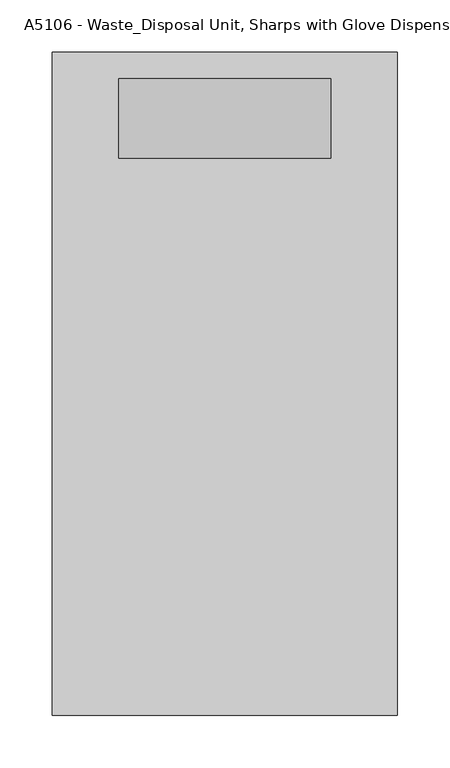
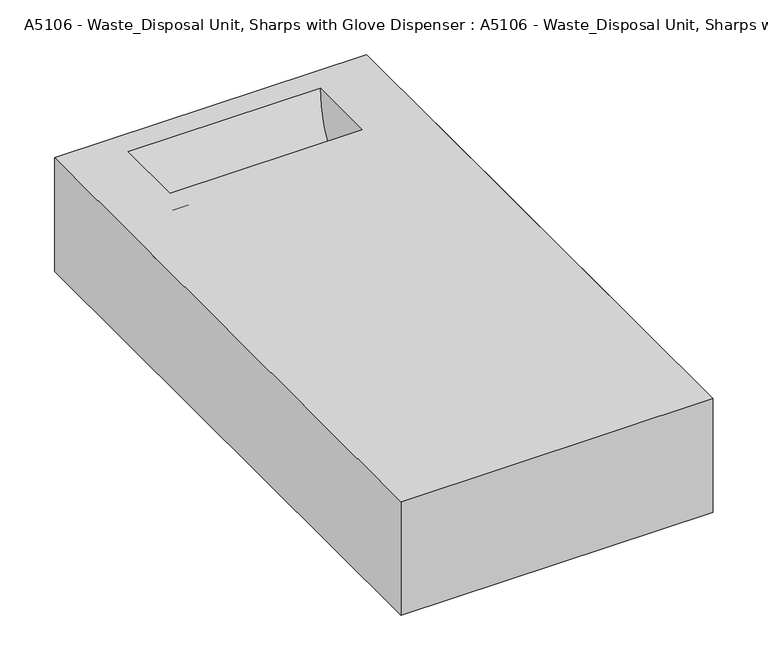
"""IFC4 building model written with IfcOpenShell, lengths in millimetres: proxy geometry, A5106 - Waste_Disposal Unit, Sharps with Glove Dispenser : A5106 - Waste_Disposal Unit, Sharps with Glove Dispenser."""

import ifcopenshell
import ifcopenshell.guid

model = None  # the IFC model being written
_history = None  # IfcOwnerHistory: only IFC2X3 demands one
_inside = {}  # id of a spatial element -> (the spatial element, [elements in it])
_under = {}  # id of a project, library or spatial element -> (it, [spatial elements below it])
_declared = {}  # id of a project -> (the project, [libraries it declares])
_typed = {}  # id of a type object -> (the type object, [elements of that type])
_made_of = {}  # id of a material, layer set ... -> (it, [elements and type objects made of it])


def new_model(schema):
    """Start an empty IFC model of exactly this schema.

    Asked for "IFC4X3", IfcOpenShell would pick the latest addendum, in which some entities
    have other attributes; the version numbers below select the first issue.
    IFC2X3 requires an IfcOwnerHistory on every rooted entity: one is made here for all.
    """
    global model, _history
    if schema == "IFC4X3":
        model = ifcopenshell.file(schema_version=(4, 3, 0, 0))
    else:
        model = ifcopenshell.file(schema=schema)
    _inside.clear()
    _under.clear()
    _declared.clear()
    _typed.clear()
    _made_of.clear()
    _history = None
    if model.schema == "IFC2X3":
        org = make("IfcOrganization", Name="unknown")
        user = make(
            "IfcPersonAndOrganization",
            ThePerson=make("IfcPerson", FamilyName="unknown"),
            TheOrganization=org,
        )
        app = make(
            "IfcApplication",
            ApplicationDeveloper=org,
            Version="unknown",
            ApplicationFullName="unknown",
            ApplicationIdentifier="unknown",
        )
        _history = make(
            "IfcOwnerHistory",
            OwningUser=user,
            OwningApplication=app,
            ChangeAction="ADDED",
            CreationDate=0,
        )
    return model


def make(cls, **values):
    """One entity of the class cls with the attributes given. An attribute that is None is left unset."""
    return model.create_entity(
        cls, **{name: value for name, value in values.items() if value is not None}
    )


def rooted(cls, **values):
    """An entity with a GlobalId (a new one), such as an element, a storey or a relation."""
    return make(cls, GlobalId=ifcopenshell.guid.new(), OwnerHistory=_history, **values)


def si_unit(unit_type, name, prefix=None):
    """IfcSIUnit, for example si_unit("LENGTHUNIT", "METRE", prefix="MILLI")."""
    return make("IfcSIUnit", UnitType=unit_type, Prefix=prefix, Name=name)


def assignment(units):
    """IfcUnitAssignment: the units of a project."""
    return None if units is None else make("IfcUnitAssignment", Units=units)


def point(xyz):
    """IfcCartesianPoint."""
    return None if xyz is None else make("IfcCartesianPoint", Coordinates=xyz)


def direction(xyz):
    """IfcDirection."""
    return None if xyz is None else make("IfcDirection", DirectionRatios=xyz)


def frame(location, z_axis=None, x_axis=None):
    """IfcAxis2Placement3D, a coordinate frame: its origin and axes. An axis left out is left unset."""
    return make(
        "IfcAxis2Placement3D",
        Location=point(location),
        Axis=direction(z_axis),
        RefDirection=direction(x_axis),
    )


def origin():
    """The frame at (0, 0, 0) with its axes left unset."""
    return frame((0.0, 0.0, 0.0))


def origin_with_axes():
    """The frame at (0, 0, 0) with the z axis (0, 0, 1) and the x axis (1, 0, 0) written out."""
    return frame((0.0, 0.0, 0.0), z_axis=(0.0, 0.0, 1.0), x_axis=(1.0, 0.0, 0.0))


def place(relative_to, where):
    """IfcLocalPlacement: puts the frame where relative to a parent placement (None: the world)."""
    return make(
        "IfcLocalPlacement", PlacementRelTo=relative_to, RelativePlacement=where
    )


def context(
    kind, dimensions, precision=None, world=None, true_north=None, identifier=None
):
    """IfcGeometricRepresentationContext, for example the 3D "Model" context."""
    return make(
        "IfcGeometricRepresentationContext",
        ContextIdentifier=identifier,
        ContextType=kind,
        CoordinateSpaceDimension=dimensions,
        Precision=precision,
        WorldCoordinateSystem=world,
        TrueNorth=true_north,
    )


def project(units=None, contexts=None):
    """IfcProject with its units and contexts."""
    return rooted(
        "IfcProject",
        Name="project",
        RepresentationContexts=contexts,
        UnitsInContext=assignment(units),
    )


def spatial(cls, under=None, at=None, **own):
    """A site, building, storey or space (cls), placed at a placement, below another one or the project."""
    s = rooted(cls, ObjectPlacement=at, **own)
    if under is not None:
        _under.setdefault(under.id(), (under, []))[1].append(s)
    return s


def polyline(points):
    """IfcPolyline through the points."""
    return make("IfcPolyline", Points=[point(p) for p in points])


def circle_curve(where, radius):
    """IfcCircle in the frame where."""
    return make("IfcCircle", Position=where, Radius=radius)


def outline(outer, holes=None, kind="AREA"):
    """IfcArbitraryClosedProfileDef: a profile drawn as a closed curve; with holes, ...WithVoids."""
    if holes is None:
        return make("IfcArbitraryClosedProfileDef", ProfileType=kind, OuterCurve=outer)
    return make(
        "IfcArbitraryProfileDefWithVoids",
        ProfileType=kind,
        OuterCurve=outer,
        InnerCurves=holes,
    )


def extrude(swept, where, along, depth):
    """IfcExtrudedAreaSolid: the profile swept, set in the frame where, extruded along a direction by depth."""
    return make(
        "IfcExtrudedAreaSolid",
        SweptArea=swept,
        Position=where,
        ExtrudedDirection=direction(along),
        Depth=depth,
    )


def shape(context_of_items, identifier, shape_type, items):
    """IfcShapeRepresentation: the items that make up one representation, for example the "Body"."""
    return make(
        "IfcShapeRepresentation",
        ContextOfItems=context_of_items,
        RepresentationIdentifier=identifier,
        RepresentationType=shape_type,
        Items=items,
    )


def source(mapping_origin, context_of_items, identifier, shape_type, items):
    """IfcRepresentationMap: a shape defined once, which mapped items show again and again."""
    return make(
        "IfcRepresentationMap",
        MappingOrigin=mapping_origin,
        MappedRepresentation=shape(context_of_items, identifier, shape_type, items),
    )


def transform(
    local_origin,
    x_axis=None,
    y_axis=None,
    z_axis=None,
    scale=None,
    scale2=None,
    scale3=None,
    uniform=True,
):
    """IfcCartesianTransformationOperator3D, or its non-uniform kind. x_axis, y_axis, z_axis: its Axis1, 2, 3."""
    if uniform:
        return make(
            "IfcCartesianTransformationOperator3D",
            Axis1=direction(x_axis),
            Axis2=direction(y_axis),
            LocalOrigin=point(local_origin),
            Scale=scale,
            Axis3=direction(z_axis),
        )
    return make(
        "IfcCartesianTransformationOperator3DnonUniform",
        Axis1=direction(x_axis),
        Axis2=direction(y_axis),
        LocalOrigin=point(local_origin),
        Scale=scale,
        Axis3=direction(z_axis),
        Scale2=scale2,
        Scale3=scale3,
    )


def mapped(mapping_source, mapping_target):
    """IfcMappedItem: shows the shape of a source again, moved by a transform."""
    return make(
        "IfcMappedItem", MappingSource=mapping_source, MappingTarget=mapping_target
    )


def made_of(thing, what):
    """Note that an element or type object is made of a material, layer set ...; save() writes the relation."""
    if what is not None:
        _made_of.setdefault(what.id(), (what, []))[1].append(thing)
    return thing


def element(
    cls,
    number,
    at=None,
    inside=None,
    cuts=None,
    type_object=None,
    material=None,
    context=None,
    identifier="Body",
    shape_type=None,
    held_by="IfcProductDefinitionShape",
    body=None,
    shapes=None,
    **own,
):
    """One element of the class cls, such as IfcWall. Its Tag is "e" and its number.

    at: its placement. inside: the storey or other place that contains it. cuts: it is an
    opening in that element (IfcRelVoidsElement). A single representation is given by context,
    identifier, shape_type and body (its items); several are given by shapes. held_by: the class
    of the entity that holds the representations. save() writes the other relations.
    """
    e = rooted(cls, Tag="e%d" % number, ObjectPlacement=at, **own)
    if body is not None:
        shapes = [shape(context, identifier, shape_type, body)]
    if shapes is not None:
        e.Representation = make(held_by, Representations=shapes)
    if inside is not None:
        _inside.setdefault(inside.id(), (inside, []))[1].append(e)
    if cuts is not None:
        rooted(
            "IfcRelVoidsElement", RelatingBuildingElement=cuts, RelatedOpeningElement=e
        )
    if type_object is not None:
        _typed.setdefault(type_object.id(), (type_object, []))[1].append(e)
    return made_of(e, material)


def aggregate(whole, parts):
    """IfcRelAggregates: a whole, such as a stair, and the parts it consists of."""
    return rooted("IfcRelAggregates", RelatingObject=whole, RelatedObjects=parts)


def save(model, path):
    """Write the relations noted so far, then the file.

    IfcRelAggregates (storeys below a building ...), IfcRelContainedInSpatialStructure (elements
    in a storey), IfcRelDefinesByType, IfcRelAssociatesMaterial and IfcRelDeclares: one each for
    every whole, place, type object, material and project.
    """
    for whole, parts in _under.values():
        aggregate(whole, parts)
    for where, things in _inside.values():
        rooted(
            "IfcRelContainedInSpatialStructure",
            RelatedElements=things,
            RelatingStructure=where,
        )
    for kind, things in _typed.values():
        rooted("IfcRelDefinesByType", RelatedObjects=things, RelatingType=kind)
    for what, things in _made_of.values():
        rooted("IfcRelAssociatesMaterial", RelatedObjects=things, RelatingMaterial=what)
    for by, libraries in _declared.values():
        rooted("IfcRelDeclares", RelatingContext=by, RelatedDefinitions=libraries)
    model.write(path)


def plane_surface(at):
    """IfcPlane: the flat surface through the origin of the frame at, square to its z axis."""
    return make("IfcPlane", Position=at)


def cylinder_surface(at, radius):
    """IfcCylindricalSurface: all points at the distance radius from the z axis of the frame at."""
    return make("IfcCylindricalSurface", Position=at, Radius=radius)


def revolved_surface(curve, axis_point, axis_direction):
    """IfcSurfaceOfRevolution: the curve turned about the line through axis_point along axis_direction."""
    return make(
        "IfcSurfaceOfRevolution",
        SweptCurve=make("IfcArbitraryOpenProfileDef", ProfileType="CURVE", Curve=curve),
        AxisPosition=make("IfcAxis1Placement", Location=point(axis_point), Axis=direction(axis_direction)),
    )


def advanced_brep(points, edges, surfaces, faces):
    """IfcAdvancedBrep: a solid bounded by faces that lie on surfaces and meet in shared edges.

    An edge is (start, end): straight between two places in points (the first is 0);
    or (start, end, curve); or (start, end, curve, False) where it runs against its curve.
    A face is (place in surfaces, loops), or (place, loops, False) where it looks against
    its surface's normal. A loop lists edges by number (the first is 1), with a minus sign
    where the edge is run from its end to its start. The first loop is the outer one.
    """
    corners = [point(p) for p in points]
    vertices = [make("IfcVertexPoint", VertexGeometry=c) for c in corners]
    made = []
    for start, end, *more in edges:
        made.append(
            make(
                "IfcEdgeCurve",
                EdgeStart=vertices[start],
                EdgeEnd=vertices[end],
                EdgeGeometry=more[0] if more else make("IfcPolyline", Points=[corners[start], corners[end]]),
                SameSense=more[1] if len(more) > 1 else True,
            )
        )
    hull = []
    for where, loops, *sense in faces:
        bounds = []
        for j, loop in enumerate(loops):
            ring = [make("IfcOrientedEdge", EdgeElement=made[abs(k) - 1], Orientation=k > 0) for k in loop]
            bounds.append(
                make(
                    "IfcFaceOuterBound" if j == 0 else "IfcFaceBound",
                    Bound=make("IfcEdgeLoop", EdgeList=ring),
                    Orientation=True,
                )
            )
        hull.append(make("IfcAdvancedFace", Bounds=bounds, FaceSurface=surfaces[where], SameSense=sense[0] if sense else True))
    return make("IfcAdvancedBrep", Outer=make("IfcClosedShell", CfsFaces=hull))


def a5106_waste_disposal_unit_sharps_with_glove_dispenser_a5106_42bc5ef0(model_context):
    return source(origin(), model_context, "Body", "SolidModel", [
        advanced_brep(
        [(101.6, 533.4, 127.0), (101.6, 457.2, 25.4), (101.6, 457.2, 127.0), (-101.6, 457.2, 127.0), (-101.6, 457.2, 25.4), (-101.6, 533.4, 127.0), (165.1, 558.8, 127.0), (-165.1, 558.8, 127.0), (-165.1, -76.2, 127.0), (165.1, -76.2, 127.0), (165.1, 558.8, 0.0), (165.1, -76.2, 0.0), (-165.1, -76.2, 0.0), (-165.1, 558.8, 0.0)],
        [
            (0, 1, circle_curve(frame((101.6, 428.5291538, 126.2781346), z_axis=(-1.0, 0.0, 0.0), x_axis=(0.0, 1.0, 0.0)), 104.8733306)),
            (1, 2),
            (2, 0),
            (3, 4),
            (4, 5, circle_curve(frame((-101.6, 428.5291538, 126.2781346), z_axis=(1.0, 0.0, 0.0), x_axis=(0.0, 1.0, 0.0)), 104.8733306)),
            (5, 3),
            (1, 4),
            (3, 2),
            (0, 5),
            (6, 7),
            (7, 8),
            (8, 9),
            (9, 6),
            (10, 11),
            (11, 12),
            (12, 13),
            (13, 10),
            (6, 10),
            (13, 7),
            (12, 8),
            (11, 9),
        ],
        [
            plane_surface(frame((101.6, 457.2, 127.0), z_axis=(-1.0, 0.0, 0.0), x_axis=(0.0, 0.0, -1.0))),
            plane_surface(frame((-101.6, 457.2, 127.0), z_axis=(1.0, 0.0, 0.0), x_axis=(0.0, 0.0, 1.0))),
            plane_surface(frame((101.6, 457.2, 127.0), z_axis=(0.0, 1.0, 0.0), x_axis=(-1.0, 0.0, 0.0))),
            revolved_surface(polyline([(101.6, 533.4024844, 126.2781346), (-101.6, 533.4024844, 126.2781346)]), (-101.6, 428.5291538, 126.2781346), (1.0, 0.0, 0.0)),
            plane_surface(frame((-165.1, 558.8, 127.0), z_axis=(0.0, 0.0, 1.0), x_axis=(-1.0, 0.0, 0.0))),
            plane_surface(frame((-165.1, 558.8, 0.0), z_axis=(0.0, 0.0, -1.0), x_axis=(1.0, 0.0, 0.0))),
            plane_surface(frame((165.1, 558.8, 127.0), z_axis=(0.0, 1.0, 0.0), x_axis=(0.0, 0.0, -1.0))),
            plane_surface(frame((-165.1, 558.8, 127.0), z_axis=(-1.0, 0.0, 0.0), x_axis=(0.0, 0.0, -1.0))),
            plane_surface(frame((-165.1, -76.2, 127.0), z_axis=(0.0, -1.0, 0.0), x_axis=(0.0, 0.0, -1.0))),
            plane_surface(frame((165.1, -76.2, 127.0), z_axis=(1.0, 0.0, 0.0), x_axis=(0.0, 0.0, -1.0))),
        ],
        [
            (0, [[1, 2, 3]]),
            (1, [[4, 5, 6]]),
            (2, [[-2, 7, -4, 8]]),
            (3, [[-1, 9, -5, -7]]),
            (4, [[10, 11, 12, 13], [-3, -8, -6, -9]]),
            (5, [[14, 15, 16, 17]]),
            (6, [[-10, 18, -17, 19]]),
            (7, [[-11, -19, -16, 20]]),
            (8, [[-12, -20, -15, 21]]),
            (9, [[-13, -21, -14, -18]]),
        ],
    ),
        advanced_brep(
        [(127.0, 431.8, 0.0), (127.0, 558.8, 127.0), (127.0, 431.8, 127.0), (-127.0, 431.8, 0.0), (-127.0, 431.8, 127.0), (-127.0, 558.8, 127.0), (101.6, 533.4, 127.0), (101.6, 457.2, 127.0), (-101.6, 457.2, 127.0), (-101.6, 533.4, 127.0), (101.6, 457.2, 25.4), (-101.6, 457.2, 25.4)],
        [
            (0, 1, circle_curve(frame((127.0, 431.8, 127.0), z_axis=(1.0, 0.0, 0.0), x_axis=(0.0, 0.0, -1.0)), 127.0)),
            (1, 2),
            (2, 0),
            (3, 4),
            (4, 5),
            (5, 3, circle_curve(frame((-127.0, 431.8, 127.0), z_axis=(-1.0, 0.0, 0.0), x_axis=(0.0, 0.0, -1.0)), 127.0)),
            (0, 3),
            (5, 1),
            (4, 2),
            (6, 7),
            (7, 8),
            (8, 9),
            (9, 6),
            (6, 10, circle_curve(frame((101.6, 428.5291538, 126.2781346), z_axis=(-1.0, 0.0, 0.0), x_axis=(0.0, 1.0, 0.0)), 104.8733306)),
            (10, 7),
            (8, 11),
            (11, 9, circle_curve(frame((-101.6, 428.5291538, 126.2781346), z_axis=(1.0, 0.0, 0.0), x_axis=(0.0, 1.0, 0.0)), 104.8733306)),
            (10, 11),
        ],
        [
            plane_surface(frame((127.0, 431.8, 0.0), z_axis=(1.0, 0.0, 0.0), x_axis=(0.0, 1.0, 0.0))),
            plane_surface(frame((-127.0, 431.8, 0.0), z_axis=(-1.0, 0.0, 0.0), x_axis=(0.0, -1.0, 0.0))),
            cylinder_surface(frame((-127.0, 431.8, 127.0), z_axis=(1.0, 0.0, 0.0), x_axis=(0.0, 0.0, -1.0)), 127.0),
            plane_surface(frame((127.0, 558.8, 127.0), z_axis=(0.0, 0.0, 1.0), x_axis=(-1.0, 0.0, 0.0))),
            plane_surface(frame((127.0, 431.8, 127.0), z_axis=(0.0, -1.0, 0.0), x_axis=(-1.0, 0.0, 0.0))),
            plane_surface(frame((101.6, 457.2, 127.0), z_axis=(-1.0, 0.0, 0.0), x_axis=(0.0, 0.0, -1.0))),
            plane_surface(frame((-101.6, 457.2, 127.0), z_axis=(1.0, 0.0, 0.0), x_axis=(0.0, 0.0, 1.0))),
            plane_surface(frame((101.6, 457.2, 127.0), z_axis=(0.0, 1.0, 0.0), x_axis=(-1.0, 0.0, 0.0))),
            revolved_surface(polyline([(101.6, 533.4024844, 126.2781346), (-101.6, 533.4024844, 126.2781346)]), (-101.6, 428.5291538, 126.2781346), (1.0, 0.0, 0.0)),
        ],
        [
            (0, [[1, 2, 3]]),
            (1, [[4, 5, 6]]),
            (2, [[-1, 7, -6, 8]]),
            (3, [[-2, -8, -5, 9], [10, 11, 12, 13]]),
            (4, [[-3, -9, -4, -7]]),
            (5, [[14, 15, -10]]),
            (6, [[16, 17, -12]]),
            (7, [[-15, 18, -16, -11]]),
            (8, [[-14, -13, -17, -18]]),
        ],
    ),
        extrude(outline(polyline([(127.0, 76.2), (127.0, -76.2), (-127.0, -76.2), (-127.0, 76.2), (127.0, 76.2)])), origin_with_axes(), (0.0, 0.0, 1.0), 101.6),
        extrude(outline(polyline([(165.1, 431.8), (165.1, 76.2), (-165.1, 76.2), (-165.1, 431.8), (165.1, 431.8)])), origin_with_axes(), (0.0, 0.0, 1.0), 127.0),
    ])


if __name__ == "__main__":
    model = new_model("IFC4")
    model_context = context("Model", 3, world=origin())
    ifc_project = project(units=[si_unit("LENGTHUNIT", "METRE", prefix="MILLI")], contexts=[model_context])
    site = spatial("IfcSite", under=ifc_project)
    building = spatial("IfcBuilding", under=site)
    placement = place(None, origin())
    a5106_waste_disposal_unit_sharps_with_glove_dispenser_a5106_shape = a5106_waste_disposal_unit_sharps_with_glove_dispenser_a5106_42bc5ef0(model_context)
    element("IfcBuildingElementProxy", 1, Name="A5106 - Waste_Disposal Unit, Sharps with Glove Dispenser : A5106 - Waste_Disposal Unit, Sharps with Glove Dispenser", ObjectType="A5106 - Waste_Disposal Unit, Sharps with Glove Dispenser : A5106 - Waste_Disposal Unit, Sharps with Glove Dispenser", at=placement, inside=building, context=model_context, shape_type="MappedRepresentation", body=[
        mapped(a5106_waste_disposal_unit_sharps_with_glove_dispenser_a5106_shape, transform((0.0, 0.0, 0.0), x_axis=(1.0, 0.0, 0.0), y_axis=(0.0, 1.0, 0.0), z_axis=(0.0, 0.0, 1.0))),
    ])
    save(model, "model.ifc")

# Revit data of these elements
# Type "A5106 - Waste_Disposal Unit, Sharps with Glove Dispenser : A5106 - Waste_Disposal Unit, Sharps with Glove Dispenser"
#   Watts2 = "0"
#   Watts1 = "0"
#   Unit_Issue = "EA"
#   UTIL_6_Misc = "-"
#   UTIL_5_NonMedGas = "-"
#   UTIL_4_MiscGas = "-"
#   UTIL_3_MedGas = "-"
#   UTIL_2_Elec = "-"
#   UTIL_1_WaterDrain = "-"
#   Nomenclature = "Waste Disposal Unit, Sharps w/Glove Dispenser"
#   NSN = "6530"
#   Location [instance default] = ""
#   JSN = "A5106"
#   Fund_Source_VA = "-"
#   Fund_Source_Navy = "-"
#   Fund_Source_Army = "-"
#   Fund_Source_AF = "-"
#   ELEC_Volts2 = "0"
#   ELEC_Volts1 = "0"
#   ELEC_Phase2 = "0"
#   ELEC_Phase1 = "0"
#   ELEC_HertzSwitch = "0"
#   ELEC_HertzDependent = "0"
#   ELEC_Hertz = "0"
#   ELEC_Amps2 = "0"
#   ELEC_Amps1 = "0"
#   DetailDescription = "The unit is designed for the disposal of sharps and complies with OSHA guidelines for the handling of sharps. It shall house a 5 quart container and be capable of being mounted on a wall. It shall have a glove dispenser attached. The unit shall be secured by a locked enclosure."
#   CAT_VA = "C"
#   CAT_Navy = "A"
#   CAT_IHS = "-"
#   CAT_Army = "C"
#   CAT_AF = "C"
#   BTUperhour = "0"
#   Weight_IP = 5
#   Default Elevation = 4' - 0"
#   DIM_Width_IP = 1' - 1"
#   DIM_Height_IP = 2' - 1"
#   DIM_Depth_IP = 0' - 5"
#   finish [instance default] = none
#   Assembly Code = ""
# Element 1 (IfcBuildingElementProxy, "A5106 - Waste_Disposal Unit, Sharps with Glove Dispenser : A5106 - Waste_Disposal Unit, Sharps with Glove Dispenser")
#   Location = "TRET3"
#   Materials on its faces: "EquipSpace"
# Materials
#   "EquipSpace": class "Unassigned", colour RGB 221 217 195, transparency 0.5
